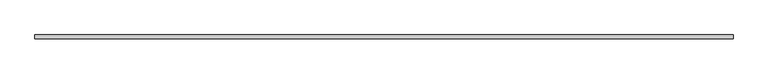
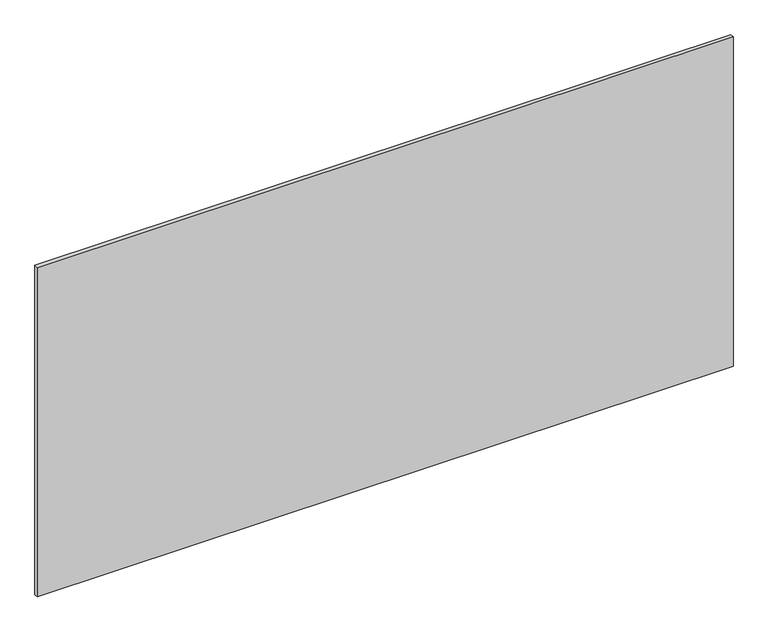
"""IFC4 building model written with IfcOpenShell, lengths in millimetres: proxy geometry, Inner panel:Inner panel:1:Inner panel:1 : Inner panel:Inner panel:300324:300043:Inner panel:1:Inner panel:1 : Inner panel:Inner panel:300324:300043 : Inner panel:Inner panel:1:Inner panel:1 : Inner panel:Inner panel:300324:300043:29 : Inner panel:Inner panel:1:Inner panel:1 : Inner panel:Inner panel:300324:300043:Inner panel:1:Inner panel:1 : Inner panel:Inner panel:300324:300043 : Inner panel:Inner panel:1:Inner panel:1 : Inner panel:Inner panel:300324:300043:300031."""

from ifc_helpers import new_model, si_unit, frame, origin, place, context, project, spatial, polyline, outline, extrude, source, transform, mapped, element, save


def generic_models_f8d5e0c5(model_context):
    return source(origin(), model_context, "Body", "SweptSolid", [
        extrude(outline(polyline([(593738.0867239, -579000.6913841), (596176.4867239, -579000.6913841), (596176.4867239, -579013.3913841), (593738.0867239, -579013.3913841), (593738.0867239, -579000.6913841)])), frame((0.0, 0.0, 2495.55), z_axis=(0.0, 0.0, 1.0), x_axis=(1.0, 0.0, 0.0)), (0.0, 0.0, 1.0), 1219.2),
    ])


if __name__ == "__main__":
    model = new_model("IFC4")
    model_context = context("Model", 3, world=origin())
    ifc_project = project(units=[si_unit("LENGTHUNIT", "METRE", prefix="MILLI")], contexts=[model_context])
    site = spatial("IfcSite", under=ifc_project)
    building = spatial("IfcBuilding", under=site)
    placement = place(None, origin())
    generic_models_shape = generic_models_f8d5e0c5(model_context)
    element("IfcBuildingElementProxy", 1, Name="Inner panel:Inner panel:1:Inner panel:1 : Inner panel:Inner panel:300324:300043:Inner panel:1:Inner panel:1 : Inner panel:Inner panel:300324:300043 : Inner panel:Inner panel:1:Inner panel:1 : Inner panel:Inner panel:300324:300043:29 : Inner panel:Inner panel:1:Inner panel:1 : Inner panel:Inner panel:300324:300043:Inner panel:1:Inner panel:1 : Inner panel:Inner panel:300324:300043 : Inner panel:Inner panel:1:Inner panel:1 : Inner panel:Inner panel:300324:300043:300031", ObjectType="Inner panel:Inner panel:1:Inner panel:1 : Inner panel:Inner panel:300324:300043:Inner panel:1:Inner panel:1 : Inner panel:Inner panel:300324:300043 : Inner panel:Inner panel:1:Inner panel:1 : Inner panel:Inner panel:300324:300043:29 : Inner panel:Inner panel:1:Inner panel:1 : Inner panel:Inner panel:300324:300043:Inner panel:1:Inner panel:1 : Inner panel:Inner panel:300324:300043 : Inner panel:Inner panel:1:Inner panel:1 : Inner panel:Inner panel:300324:300043:300031", at=placement, inside=building, context=model_context, shape_type="MappedRepresentation", body=[
        mapped(generic_models_shape, transform((0.0, 0.0, 0.0), x_axis=(1.0, 0.0, 0.0), y_axis=(0.0, 1.0, 0.0), z_axis=(0.0, 0.0, 1.0))),
    ])
    save(model, "model.ifc")

# Revit data of these elements
# Type "Inner panel:Inner panel:1:Inner panel:1 : Inner panel:Inner panel:300324:300043:Inner panel:1:Inner panel:1 : Inner panel:Inner panel:300324:300043 : Inner panel:Inner panel:1:Inner panel:1 : Inner panel:Inner panel:300324:300043:29 : Inner panel:Inner panel:1:Inner panel:1 : Inner panel:Inner panel:300324:300043:Inner panel:1:Inner panel:1 : Inner panel:Inner panel:300324:300043 : Inner panel:Inner panel:1:Inner panel:1 : Inner panel:Inner panel:300324:300043:300031"
#   NameOverride = "Inner panel:Inner panel:1:Inner panel:1 : Inner panel:Inner panel:300324:300043:Inner panel:1:Inner panel:1 : Inner panel:Inner panel:300324:300043 : Inner panel:Inner panel:1:Inner panel:1 : Inner panel:Inner panel:300324:300043:300031"
#   ObjectTypeOverride = "Inner panel:1:Inner panel:1 : Inner panel:Inner panel:300324:300043 : Inner panel:Inner panel:1:Inner panel:1 : Inner panel:Inner panel:300324:300043"
#   Reference = "Inner panel"
#   Tag = "300031"
# Element 1 (IfcBuildingElementProxy, "Inner panel:Inner panel:1:Inner panel:1 : Inner panel:Inner panel:300324:300043:Inner panel:1:Inner panel:1 : Inner panel:Inner panel:300324:300043 : Inner panel:Inner panel:1:Inner panel:1 : Inner panel:Inner panel:300324:300043:29 : Inner panel:Inner panel:1:Inner panel:1 : Inner panel:Inner panel:300324:300043:Inner panel:1:Inner panel:1 : Inner panel:Inner panel:300324:300043 : Inner panel:Inner panel:1:Inner panel:1 : Inner panel:Inner panel:300324:300043:300031")
#   Materials on its faces: "1/2\" EXTERIOR GRADE FIRE RETARDANT CDX PLYWOOD"
# Materials
#   "1/2\" EXTERIOR GRADE FIRE RETARDANT CDX PLYWOOD": class "Unassigned", colour RGB 196 177 123, transparency 0, Cost = 0
